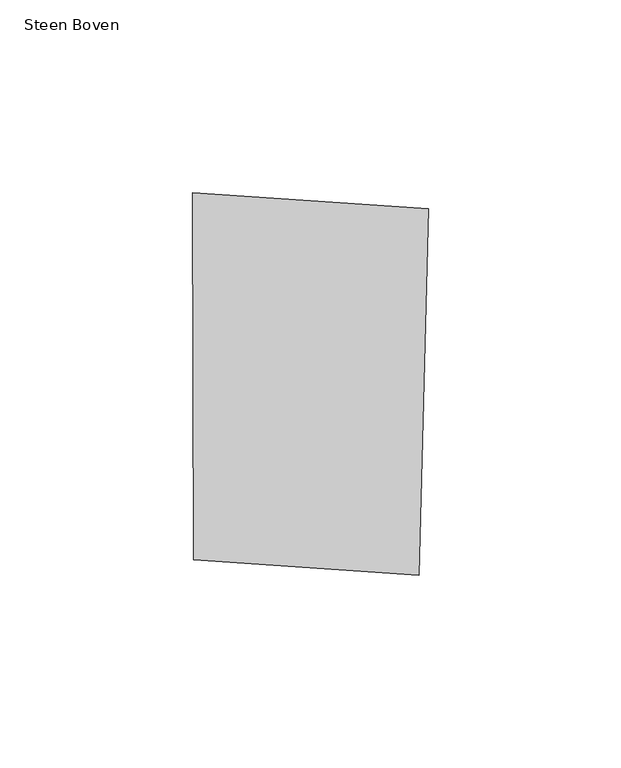
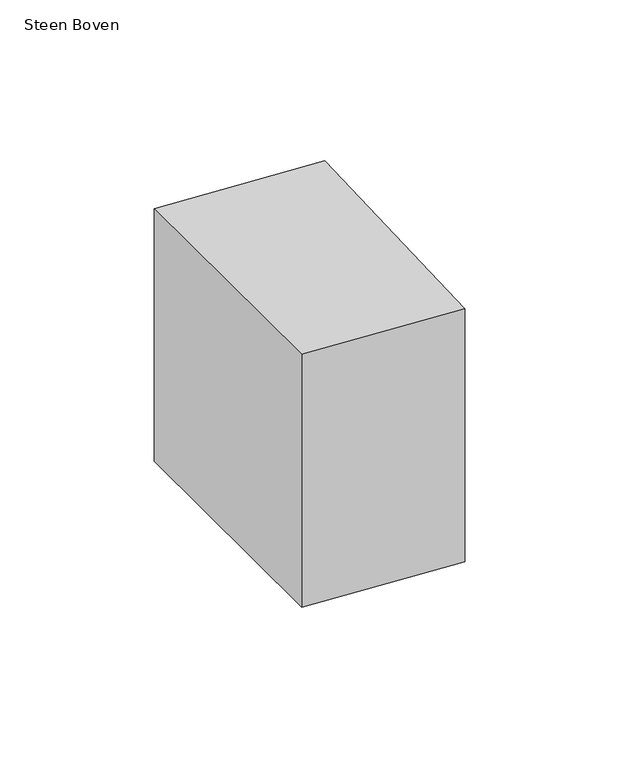
"""IFC4 building model written with IfcOpenShell, lengths in millimetres: proxy geometry, 00_GMA_steen_versie_4 : Steen Boven."""

from ifc_helpers import new_model, si_unit, origin, origin_with_axes, place, context, project, spatial, polyline, outline, extrude, source, transform, mapped, element, save


def steen_boven_c9ed0400(model_context):
    return source(origin(), model_context, "Body", "SweptSolid", [
        extrude(outline(polyline([(101.8711208, 118.9695374), (99.38934, 23.9095435), (40.8147254, 27.9466758), (40.5884353, 123.200595), (101.8711208, 118.9695374)])), origin_with_axes(), (0.0, 0.0, 1.0), 100.0),
    ])


if __name__ == "__main__":
    model = new_model("IFC4")
    model_context = context("Model", 3, world=origin())
    ifc_project = project(units=[si_unit("LENGTHUNIT", "METRE", prefix="MILLI")], contexts=[model_context])
    site = spatial("IfcSite", under=ifc_project)
    building = spatial("IfcBuilding", under=site)
    placement = place(None, origin())
    steen_boven_shape = steen_boven_c9ed0400(model_context)
    element("IfcBuildingElementProxy", 1, Name="00_GMA_steen_versie_4 : Steen Boven", ObjectType="00_GMA_steen_versie_4 : Steen Boven", at=placement, inside=building, context=model_context, shape_type="MappedRepresentation", body=[
        mapped(steen_boven_shape, transform((0.0, 0.0, 0.0), x_axis=(1.0, 0.0, 0.0), y_axis=(0.0, 1.0, 0.0), z_axis=(0.0, 0.0, 1.0))),
    ])
    save(model, "model.ifc")

# Revit data of these elements
# Type "00_GMA_steen_versie_4 : Steen Boven"
#   StootVoegHalfBoven [instance default] = 5 mm
#   StootVoegHalf [instance default] = 5 mm
#   StootVoegBreedteOnder = 10 mm
#   StootVoegBreedteBoven = 10 mm
#   Steendikte = 100 mm
#   LintVoegOnderHalf = 5 mm
#   LintVoegOnder = 10 mm
#   LintVoegBovenHalf = 0 mm
#   LintVoegBoven = 0 mm
#   materiaal = none
#   MateriaalVoeg = none
#   Default Elevation = 0
